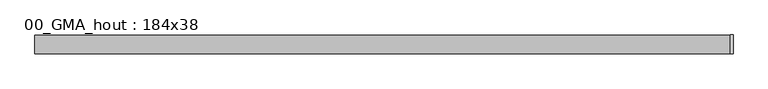
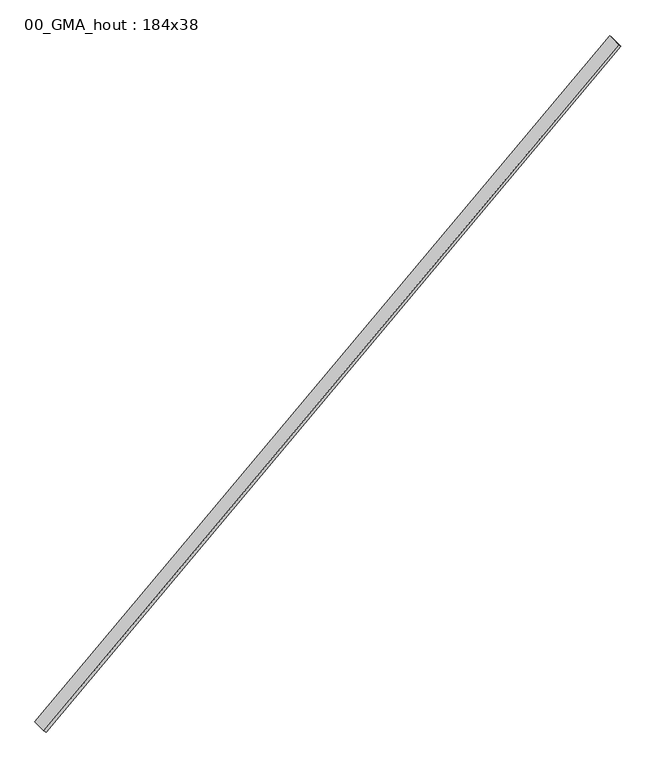
"""IFC4 building model written with IfcOpenShell, lengths in millimetres: proxy geometry, 00_GMA_hout : 184x38."""

import ifcopenshell
import ifcopenshell.guid

model = None  # the IFC model being written
_history = None  # IfcOwnerHistory: only IFC2X3 demands one
_inside = {}  # id of a spatial element -> (the spatial element, [elements in it])
_under = {}  # id of a project, library or spatial element -> (it, [spatial elements below it])
_declared = {}  # id of a project -> (the project, [libraries it declares])
_typed = {}  # id of a type object -> (the type object, [elements of that type])
_made_of = {}  # id of a material, layer set ... -> (it, [elements and type objects made of it])


def new_model(schema):
    """Start an empty IFC model of exactly this schema.

    Asked for "IFC4X3", IfcOpenShell would pick the latest addendum, in which some entities
    have other attributes; the version numbers below select the first issue.
    IFC2X3 requires an IfcOwnerHistory on every rooted entity: one is made here for all.
    """
    global model, _history
    if schema == "IFC4X3":
        model = ifcopenshell.file(schema_version=(4, 3, 0, 0))
    else:
        model = ifcopenshell.file(schema=schema)
    _inside.clear()
    _under.clear()
    _declared.clear()
    _typed.clear()
    _made_of.clear()
    _history = None
    if model.schema == "IFC2X3":
        org = make("IfcOrganization", Name="unknown")
        user = make(
            "IfcPersonAndOrganization",
            ThePerson=make("IfcPerson", FamilyName="unknown"),
            TheOrganization=org,
        )
        app = make(
            "IfcApplication",
            ApplicationDeveloper=org,
            Version="unknown",
            ApplicationFullName="unknown",
            ApplicationIdentifier="unknown",
        )
        _history = make(
            "IfcOwnerHistory",
            OwningUser=user,
            OwningApplication=app,
            ChangeAction="ADDED",
            CreationDate=0,
        )
    return model


def make(cls, **values):
    """One entity of the class cls with the attributes given. An attribute that is None is left unset."""
    return model.create_entity(
        cls, **{name: value for name, value in values.items() if value is not None}
    )


def rooted(cls, **values):
    """An entity with a GlobalId (a new one), such as an element, a storey or a relation."""
    return make(cls, GlobalId=ifcopenshell.guid.new(), OwnerHistory=_history, **values)


def si_unit(unit_type, name, prefix=None):
    """IfcSIUnit, for example si_unit("LENGTHUNIT", "METRE", prefix="MILLI")."""
    return make("IfcSIUnit", UnitType=unit_type, Prefix=prefix, Name=name)


def assignment(units):
    """IfcUnitAssignment: the units of a project."""
    return None if units is None else make("IfcUnitAssignment", Units=units)


def point(xyz):
    """IfcCartesianPoint."""
    return None if xyz is None else make("IfcCartesianPoint", Coordinates=xyz)


def direction(xyz):
    """IfcDirection."""
    return None if xyz is None else make("IfcDirection", DirectionRatios=xyz)


def frame(location, z_axis=None, x_axis=None):
    """IfcAxis2Placement3D, a coordinate frame: its origin and axes. An axis left out is left unset."""
    return make(
        "IfcAxis2Placement3D",
        Location=point(location),
        Axis=direction(z_axis),
        RefDirection=direction(x_axis),
    )


def origin():
    """The frame at (0, 0, 0) with its axes left unset."""
    return frame((0.0, 0.0, 0.0))


def place(relative_to, where):
    """IfcLocalPlacement: puts the frame where relative to a parent placement (None: the world)."""
    return make(
        "IfcLocalPlacement", PlacementRelTo=relative_to, RelativePlacement=where
    )


def context(
    kind, dimensions, precision=None, world=None, true_north=None, identifier=None
):
    """IfcGeometricRepresentationContext, for example the 3D "Model" context."""
    return make(
        "IfcGeometricRepresentationContext",
        ContextIdentifier=identifier,
        ContextType=kind,
        CoordinateSpaceDimension=dimensions,
        Precision=precision,
        WorldCoordinateSystem=world,
        TrueNorth=true_north,
    )


def project(units=None, contexts=None):
    """IfcProject with its units and contexts."""
    return rooted(
        "IfcProject",
        Name="project",
        RepresentationContexts=contexts,
        UnitsInContext=assignment(units),
    )


def spatial(cls, under=None, at=None, **own):
    """A site, building, storey or space (cls), placed at a placement, below another one or the project."""
    s = rooted(cls, ObjectPlacement=at, **own)
    if under is not None:
        _under.setdefault(under.id(), (under, []))[1].append(s)
    return s


def polyline(points):
    """IfcPolyline through the points."""
    return make("IfcPolyline", Points=[point(p) for p in points])


def outline(outer, holes=None, kind="AREA"):
    """IfcArbitraryClosedProfileDef: a profile drawn as a closed curve; with holes, ...WithVoids."""
    if holes is None:
        return make("IfcArbitraryClosedProfileDef", ProfileType=kind, OuterCurve=outer)
    return make(
        "IfcArbitraryProfileDefWithVoids",
        ProfileType=kind,
        OuterCurve=outer,
        InnerCurves=holes,
    )


def extrude(swept, where, along, depth):
    """IfcExtrudedAreaSolid: the profile swept, set in the frame where, extruded along a direction by depth."""
    return make(
        "IfcExtrudedAreaSolid",
        SweptArea=swept,
        Position=where,
        ExtrudedDirection=direction(along),
        Depth=depth,
    )


def shape(context_of_items, identifier, shape_type, items):
    """IfcShapeRepresentation: the items that make up one representation, for example the "Body"."""
    return make(
        "IfcShapeRepresentation",
        ContextOfItems=context_of_items,
        RepresentationIdentifier=identifier,
        RepresentationType=shape_type,
        Items=items,
    )


def source(mapping_origin, context_of_items, identifier, shape_type, items):
    """IfcRepresentationMap: a shape defined once, which mapped items show again and again."""
    return make(
        "IfcRepresentationMap",
        MappingOrigin=mapping_origin,
        MappedRepresentation=shape(context_of_items, identifier, shape_type, items),
    )


def transform(
    local_origin,
    x_axis=None,
    y_axis=None,
    z_axis=None,
    scale=None,
    scale2=None,
    scale3=None,
    uniform=True,
):
    """IfcCartesianTransformationOperator3D, or its non-uniform kind. x_axis, y_axis, z_axis: its Axis1, 2, 3."""
    if uniform:
        return make(
            "IfcCartesianTransformationOperator3D",
            Axis1=direction(x_axis),
            Axis2=direction(y_axis),
            LocalOrigin=point(local_origin),
            Scale=scale,
            Axis3=direction(z_axis),
        )
    return make(
        "IfcCartesianTransformationOperator3DnonUniform",
        Axis1=direction(x_axis),
        Axis2=direction(y_axis),
        LocalOrigin=point(local_origin),
        Scale=scale,
        Axis3=direction(z_axis),
        Scale2=scale2,
        Scale3=scale3,
    )


def mapped(mapping_source, mapping_target):
    """IfcMappedItem: shows the shape of a source again, moved by a transform."""
    return make(
        "IfcMappedItem", MappingSource=mapping_source, MappingTarget=mapping_target
    )


def made_of(thing, what):
    """Note that an element or type object is made of a material, layer set ...; save() writes the relation."""
    if what is not None:
        _made_of.setdefault(what.id(), (what, []))[1].append(thing)
    return thing


def element(
    cls,
    number,
    at=None,
    inside=None,
    cuts=None,
    type_object=None,
    material=None,
    context=None,
    identifier="Body",
    shape_type=None,
    held_by="IfcProductDefinitionShape",
    body=None,
    shapes=None,
    **own,
):
    """One element of the class cls, such as IfcWall. Its Tag is "e" and its number.

    at: its placement. inside: the storey or other place that contains it. cuts: it is an
    opening in that element (IfcRelVoidsElement). A single representation is given by context,
    identifier, shape_type and body (its items); several are given by shapes. held_by: the class
    of the entity that holds the representations. save() writes the other relations.
    """
    e = rooted(cls, Tag="e%d" % number, ObjectPlacement=at, **own)
    if body is not None:
        shapes = [shape(context, identifier, shape_type, body)]
    if shapes is not None:
        e.Representation = make(held_by, Representations=shapes)
    if inside is not None:
        _inside.setdefault(inside.id(), (inside, []))[1].append(e)
    if cuts is not None:
        rooted(
            "IfcRelVoidsElement", RelatingBuildingElement=cuts, RelatedOpeningElement=e
        )
    if type_object is not None:
        _typed.setdefault(type_object.id(), (type_object, []))[1].append(e)
    return made_of(e, material)


def aggregate(whole, parts):
    """IfcRelAggregates: a whole, such as a stair, and the parts it consists of."""
    return rooted("IfcRelAggregates", RelatingObject=whole, RelatedObjects=parts)


def save(model, path):
    """Write the relations noted so far, then the file.

    IfcRelAggregates (storeys below a building ...), IfcRelContainedInSpatialStructure (elements
    in a storey), IfcRelDefinesByType, IfcRelAssociatesMaterial and IfcRelDeclares: one each for
    every whole, place, type object, material and project.
    """
    for whole, parts in _under.values():
        aggregate(whole, parts)
    for where, things in _inside.values():
        rooted(
            "IfcRelContainedInSpatialStructure",
            RelatedElements=things,
            RelatingStructure=where,
        )
    for kind, things in _typed.values():
        rooted("IfcRelDefinesByType", RelatedObjects=things, RelatingType=kind)
    for what, things in _made_of.values():
        rooted("IfcRelAssociatesMaterial", RelatedObjects=things, RelatingMaterial=what)
    for by, libraries in _declared.values():
        rooted("IfcRelDeclares", RelatingContext=by, RelatedDefinitions=libraries)
    model.write(path)


def proxy_00_gma_hout_184x38_33489daf(model_context):
    return source(origin(), model_context, "Body", "SweptSolid", [
        extrude(outline(polyline([(-92.0, 0.0), (92.0, 0.0), (92.0, -9193.2589371), (-92.0, -9193.2589371), (-92.0, 0.0)])), frame((-2954.4726009, -92.0, -2692.5027766), z_axis=(-0.67357883778224, 0.0, 0.7391153829355244), x_axis=(0.0, 1.0, 0.0)), (0.0, 0.0, 1.0), 38.0),
    ])


if __name__ == "__main__":
    model = new_model("IFC4")
    model_context = context("Model", 3, world=origin())
    ifc_project = project(units=[si_unit("LENGTHUNIT", "METRE", prefix="MILLI")], contexts=[model_context])
    site = spatial("IfcSite", under=ifc_project)
    building = spatial("IfcBuilding", under=site)
    placement = place(None, origin())
    proxy_00_gma_hout_184x38_shape = proxy_00_gma_hout_184x38_33489daf(model_context)
    element("IfcBuildingElementProxy", 1, Name="00_GMA_hout : 184x38", ObjectType="00_GMA_hout : 184x38", at=placement, inside=building, context=model_context, shape_type="MappedRepresentation", body=[
        mapped(proxy_00_gma_hout_184x38_shape, transform((0.0, 0.0, 0.0), x_axis=(1.0, 0.0, 0.0), y_axis=(0.0, 1.0, 0.0), z_axis=(0.0, 0.0, 1.0))),
    ])
    save(model, "model.ifc")

# Revit data of these elements
# Type "00_GMA_hout : 184x38"
#   lengte [instance default] = 1198.641 mm
#   h = 38 mm
#   b = 184 mm
#   materiaal = 00_hout_vuren_generiek
#   PositionProfile [instance default] = 00_GMP_rectangle : TopLeft
#   Default Elevation = 0
# Element 1 (IfcBuildingElementProxy, "00_GMA_hout : 184x38")
#   lengte = 9193.259 mm
#   PositionProfile = 00_GMP_rectangle : BottomRight
#   Materials on its faces: "00_hout_vuren_generiek"
# Materials
#   "00_hout_vuren_generiek": class "Wood", colour RGB 255 128 0, transparency 0, Manufacturer = "RevitGG", URL = "www.revitgg.nl", Description = "Hout, vuren, generiek", Cost = 0
